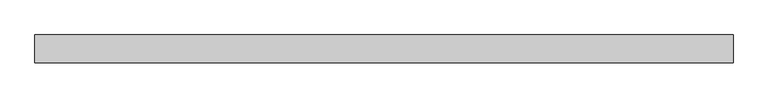
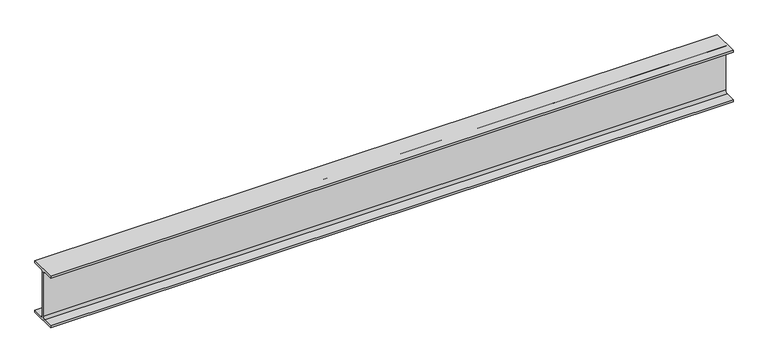
"""IFC4 building model written with IfcOpenShell, lengths in millimetres: beam geometry, 0912_Steel Framing_H-KSD3502 : H_SB_ASB_H-250x125x6x9."""

from ifc_helpers import new_model, si_unit, point, frame, frame_2d, origin, place, context, project, spatial, polyline, circle_curve, trimmed, segment, composite_curve, outline, extrude, source, transform, mapped, element, save


def beam_fa849394(model_context):
    return source(origin(), model_context, "Body", "SweptSolid", [
        extrude(outline(composite_curve([segment(polyline([(62.5, -116.0), (62.5, -125.0), (-62.5, -125.0), (-62.5, -116.0), (-15.0, -116.0)]), True, "CONTINUOUS"), segment(trimmed(circle_curve(frame_2d((-15.0, -104.0)), 12.0), [point((-15.0, -116.0))], [point((-3.0, -104.0))], True, "CARTESIAN"), True, "CONTINUOUS"), segment(polyline([(-3.0, -104.0), (-3.0, 104.0)]), True, "CONTINUOUS"), segment(trimmed(circle_curve(frame_2d((-15.0, 104.0)), 12.0), [point((-3.0, 104.0))], [point((-15.0, 116.0))], True, "CARTESIAN"), True, "CONTINUOUS"), segment(polyline([(-15.0, 116.0), (-62.5, 116.0), (-62.5, 125.0), (62.5, 125.0), (62.5, 116.0), (15.0, 116.0)]), True, "CONTINUOUS"), segment(trimmed(circle_curve(frame_2d((15.0, 104.0)), 12.0), [point((15.0, 116.0))], [point((3.0, 104.0))], True, "CARTESIAN"), True, "CONTINUOUS"), segment(polyline([(3.0, 104.0), (3.0, -104.0)]), True, "CONTINUOUS"), segment(trimmed(circle_curve(frame_2d((15.0, -104.0)), 12.0), [point((3.0, -104.0))], [point((15.0, -116.0))], True, "CARTESIAN"), True, "CONTINUOUS"), segment(polyline([(15.0, -116.0), (62.5, -116.0)]), True, "CONTINUOUS")], self_intersect=False)), frame((-1494.5360727, 0.0, 0.0), z_axis=(1.0, 0.0, 0.0), x_axis=(0.0, 1.0, 0.0)), (0.0, 0.0, 1.0), 3149.3360727),
    ])


if __name__ == "__main__":
    model = new_model("IFC4")
    model_context = context("Model", 3, world=origin())
    ifc_project = project(units=[si_unit("LENGTHUNIT", "METRE", prefix="MILLI")], contexts=[model_context])
    site = spatial("IfcSite", under=ifc_project)
    building = spatial("IfcBuilding", under=site)
    placement = place(None, origin())
    beam_shape = beam_fa849394(model_context)
    element("IfcBeam", 1, ObjectType="0912_Steel Framing_H-KSD3502 : H_SB_ASB_H-250x125x6x9", at=placement, inside=building, context=model_context, shape_type="MappedRepresentation", body=[
        mapped(beam_shape, transform((0.0, 0.0, 0.0), x_axis=(1.0, 0.0, 0.0), y_axis=(0.0, 1.0, 0.0), z_axis=(0.0, 0.0, 1.0))),
    ])
    save(model, "model.ifc")

# Revit data of these elements
# Type "0912_Steel Framing_H-KSD3502 : H_SB_ASB_H-250x125x6x9"
#   H_WM Code_1 = "S01AA003-00001 | Main Steel Structure Fabrication Work | Shelter/Building | Light Steel - Standard (30KG/M>Weight) | Material: (   )"
#   H_WM Code_2 = "S03AA029-00001 | Main Steel Structure Erection Work | Shelter/Building | Light Steel (30KG/M>Weight) | Material: (   )"
#   H_WM Code_3 = "S01AA010-00001 | Main Steel Structure Fabrication Work | Shelter/Building | Steel Painting/Coating | for Non-Fireproofed Steel Surface, Surface Preparation, Primer, Second & Final Coat | Material: (   )"
#   H_Q'ty Cal Type Tag = "SB-Q2"
#   Width = 12.5 cm
#   Web Thickness = 0.6 cm
#   Web Fillet = 1.2 cm
#   Warping Constant = 42539.8 cm⁶
#   W = 0
#   Torsional Moment of Inertia = 7.8102 cm⁴
#   Section Area = 37.66 cm²
#   Plastic Modulus weak axis = 73.1 cm³
#   Plastic Modulus strong axis = 366.0 cm³
#   Perimeter = 0.97 m²/m
#   Nominal Weight = 29.60 kgf/m
#   Moment of Inertia weak axis = 294.00 cm⁴
#   Moment of Inertia strong axis = 4050.00 cm⁴
#   Height = 25.0 cm
#   Flange Thickness = 0.9 cm
#   Elastic Modulus weak axis = 47.0 cm³
#   Elastic Modulus strong axis = 324.0 cm³
#   Centroid Vertical = 12.5 cm
#   Centroid Horizontal = 6.25 cm
#   Ix = 40500000
#   Length [instance default] = 1.5240 m
#   Zx = 366000
#   b = 0.1250 m
#   h = 0.2500 m
#   r = 0.0120 m
#   s = 0.0060 m
#   t = 0.0090 m
#   A = 0.003766 m²
#   Structural Material [instance default] = Steel, 45-345
#   Assembly Code = ""
# Element 1 (IfcBeam, "0912_Steel Framing_H-KSD3502 : H_SB_ASB_H-250x125x6x9")
#   Structural Material = none
# Materials
#   "Steel, 45-345": class "Metal", colour RGB 189 187 185, transparency 0, Description = "Steel 345 MPa", Cost = 0
